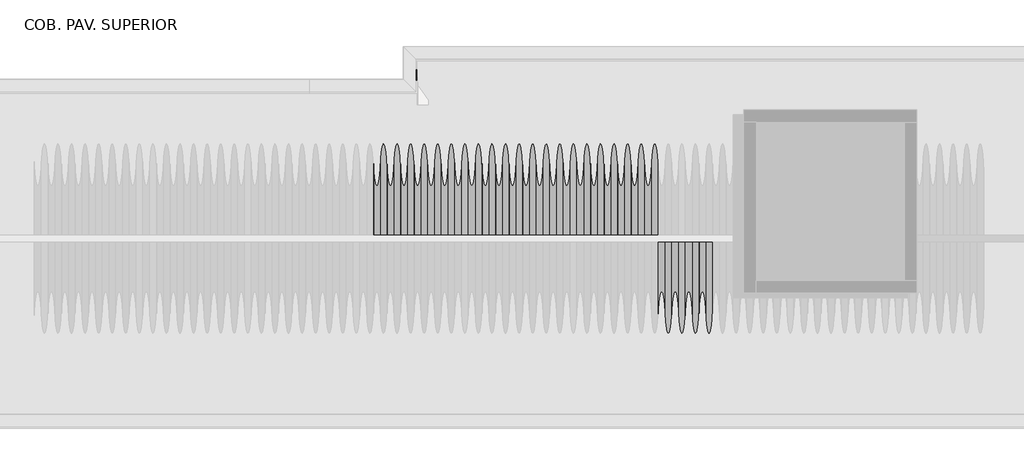
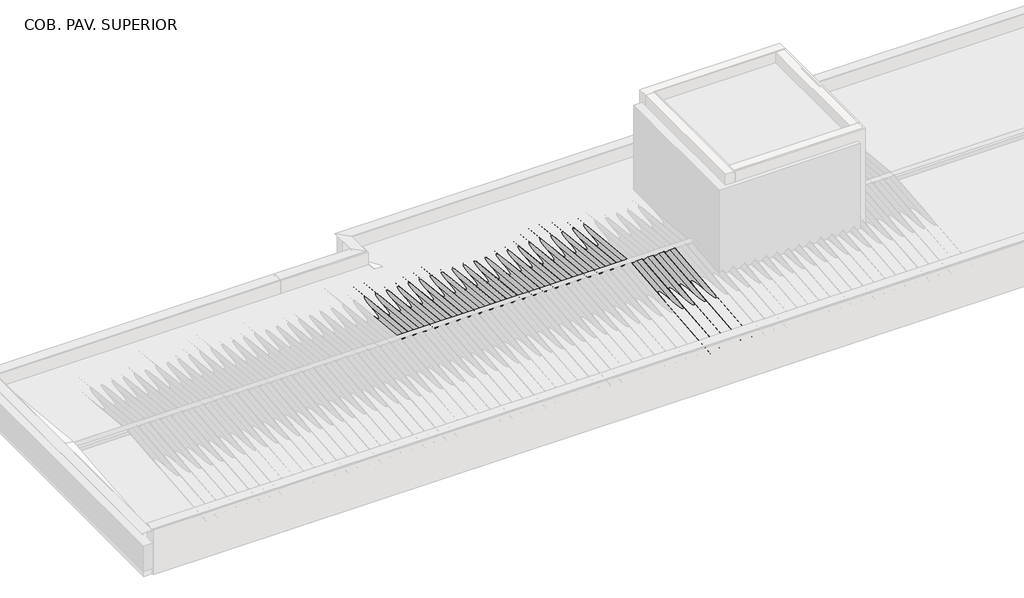
# One storey, part 5 of 8: 37 beams, 12 columns.
"""IFC4 building model written with IfcOpenShell, lengths in millimetres."""

import ifcopenshell
import ifcopenshell.guid

model = None  # the IFC model being written
_history = None  # IfcOwnerHistory: only IFC2X3 demands one
_inside = {}  # id of a spatial element -> (the spatial element, [elements in it])
_under = {}  # id of a project, library or spatial element -> (it, [spatial elements below it])
_declared = {}  # id of a project -> (the project, [libraries it declares])
_typed = {}  # id of a type object -> (the type object, [elements of that type])
_made_of = {}  # id of a material, layer set ... -> (it, [elements and type objects made of it])


def new_model(schema):
    """Start an empty IFC model of exactly this schema.

    Asked for "IFC4X3", IfcOpenShell would pick the latest addendum, in which some entities
    have other attributes; the version numbers below select the first issue.
    IFC2X3 requires an IfcOwnerHistory on every rooted entity: one is made here for all.
    """
    global model, _history
    if schema == "IFC4X3":
        model = ifcopenshell.file(schema_version=(4, 3, 0, 0))
    else:
        model = ifcopenshell.file(schema=schema)
    _inside.clear()
    _under.clear()
    _declared.clear()
    _typed.clear()
    _made_of.clear()
    _history = None
    if model.schema == "IFC2X3":
        org = make("IfcOrganization", Name="unknown")
        user = make(
            "IfcPersonAndOrganization",
            ThePerson=make("IfcPerson", FamilyName="unknown"),
            TheOrganization=org,
        )
        app = make(
            "IfcApplication",
            ApplicationDeveloper=org,
            Version="unknown",
            ApplicationFullName="unknown",
            ApplicationIdentifier="unknown",
        )
        _history = make(
            "IfcOwnerHistory",
            OwningUser=user,
            OwningApplication=app,
            ChangeAction="ADDED",
            CreationDate=0,
        )
    return model


def make(cls, **values):
    """One entity of the class cls with the attributes given. An attribute that is None is left unset."""
    return model.create_entity(
        cls, **{name: value for name, value in values.items() if value is not None}
    )


def rooted(cls, **values):
    """An entity with a GlobalId (a new one), such as an element, a storey or a relation."""
    return make(cls, GlobalId=ifcopenshell.guid.new(), OwnerHistory=_history, **values)


def si_unit(unit_type, name, prefix=None):
    """IfcSIUnit, for example si_unit("LENGTHUNIT", "METRE", prefix="MILLI")."""
    return make("IfcSIUnit", UnitType=unit_type, Prefix=prefix, Name=name)


def assignment(units):
    """IfcUnitAssignment: the units of a project."""
    return None if units is None else make("IfcUnitAssignment", Units=units)


def point(xyz):
    """IfcCartesianPoint."""
    return None if xyz is None else make("IfcCartesianPoint", Coordinates=xyz)


def direction(xyz):
    """IfcDirection."""
    return None if xyz is None else make("IfcDirection", DirectionRatios=xyz)


def frame(location, z_axis=None, x_axis=None):
    """IfcAxis2Placement3D, a coordinate frame: its origin and axes. An axis left out is left unset."""
    return make(
        "IfcAxis2Placement3D",
        Location=point(location),
        Axis=direction(z_axis),
        RefDirection=direction(x_axis),
    )


def frame_2d(location, x_axis=None):
    """IfcAxis2Placement2D, a coordinate frame in the plane: its origin and x axis."""
    return make(
        "IfcAxis2Placement2D", Location=point(location), RefDirection=direction(x_axis)
    )


def origin():
    """The frame at (0, 0, 0) with its axes left unset."""
    return frame((0.0, 0.0, 0.0))


def place(relative_to, where):
    """IfcLocalPlacement: puts the frame where relative to a parent placement (None: the world)."""
    return make(
        "IfcLocalPlacement", PlacementRelTo=relative_to, RelativePlacement=where
    )


def context(
    kind, dimensions, precision=None, world=None, true_north=None, identifier=None
):
    """IfcGeometricRepresentationContext, for example the 3D "Model" context."""
    return make(
        "IfcGeometricRepresentationContext",
        ContextIdentifier=identifier,
        ContextType=kind,
        CoordinateSpaceDimension=dimensions,
        Precision=precision,
        WorldCoordinateSystem=world,
        TrueNorth=true_north,
    )


def project(units=None, contexts=None):
    """IfcProject with its units and contexts."""
    return rooted(
        "IfcProject",
        Name="project",
        RepresentationContexts=contexts,
        UnitsInContext=assignment(units),
    )


def spatial(cls, under=None, at=None, **own):
    """A site, building, storey or space (cls), placed at a placement, below another one or the project."""
    s = rooted(cls, ObjectPlacement=at, **own)
    if under is not None:
        _under.setdefault(under.id(), (under, []))[1].append(s)
    return s


def polyline(points):
    """IfcPolyline through the points."""
    return make("IfcPolyline", Points=[point(p) for p in points])


def circle_curve(where, radius):
    """IfcCircle in the frame where."""
    return make("IfcCircle", Position=where, Radius=radius)


def trimmed(basis, trim1, trim2, sense, master):
    """IfcTrimmedCurve: the piece of a basis curve between two trims."""
    return make(
        "IfcTrimmedCurve",
        BasisCurve=basis,
        Trim1=trim1,
        Trim2=trim2,
        SenseAgreement=sense,
        MasterRepresentation=master,
    )


def segment(curve, same_sense, transition):
    """IfcCompositeCurveSegment."""
    return make(
        "IfcCompositeCurveSegment",
        Transition=transition,
        SameSense=same_sense,
        ParentCurve=curve,
    )


def composite_curve(segments, self_intersect=None):
    """IfcCompositeCurve: segments joined end to end."""
    return make("IfcCompositeCurve", Segments=segments, SelfIntersect=self_intersect)


def outline(outer, holes=None, kind="AREA"):
    """IfcArbitraryClosedProfileDef: a profile drawn as a closed curve; with holes, ...WithVoids."""
    if holes is None:
        return make("IfcArbitraryClosedProfileDef", ProfileType=kind, OuterCurve=outer)
    return make(
        "IfcArbitraryProfileDefWithVoids",
        ProfileType=kind,
        OuterCurve=outer,
        InnerCurves=holes,
    )


def extrude(swept, where, along, depth):
    """IfcExtrudedAreaSolid: the profile swept, set in the frame where, extruded along a direction by depth."""
    return make(
        "IfcExtrudedAreaSolid",
        SweptArea=swept,
        Position=where,
        ExtrudedDirection=direction(along),
        Depth=depth,
    )


def shape(context_of_items, identifier, shape_type, items):
    """IfcShapeRepresentation: the items that make up one representation, for example the "Body"."""
    return make(
        "IfcShapeRepresentation",
        ContextOfItems=context_of_items,
        RepresentationIdentifier=identifier,
        RepresentationType=shape_type,
        Items=items,
    )


def source(mapping_origin, context_of_items, identifier, shape_type, items):
    """IfcRepresentationMap: a shape defined once, which mapped items show again and again."""
    return make(
        "IfcRepresentationMap",
        MappingOrigin=mapping_origin,
        MappedRepresentation=shape(context_of_items, identifier, shape_type, items),
    )


def transform(
    local_origin,
    x_axis=None,
    y_axis=None,
    z_axis=None,
    scale=None,
    scale2=None,
    scale3=None,
    uniform=True,
):
    """IfcCartesianTransformationOperator3D, or its non-uniform kind. x_axis, y_axis, z_axis: its Axis1, 2, 3."""
    if uniform:
        return make(
            "IfcCartesianTransformationOperator3D",
            Axis1=direction(x_axis),
            Axis2=direction(y_axis),
            LocalOrigin=point(local_origin),
            Scale=scale,
            Axis3=direction(z_axis),
        )
    return make(
        "IfcCartesianTransformationOperator3DnonUniform",
        Axis1=direction(x_axis),
        Axis2=direction(y_axis),
        LocalOrigin=point(local_origin),
        Scale=scale,
        Axis3=direction(z_axis),
        Scale2=scale2,
        Scale3=scale3,
    )


def mapped(mapping_source, mapping_target):
    """IfcMappedItem: shows the shape of a source again, moved by a transform."""
    return make(
        "IfcMappedItem", MappingSource=mapping_source, MappingTarget=mapping_target
    )


def made_of(thing, what):
    """Note that an element or type object is made of a material, layer set ...; save() writes the relation."""
    if what is not None:
        _made_of.setdefault(what.id(), (what, []))[1].append(thing)
    return thing


def element(
    cls,
    number,
    at=None,
    inside=None,
    cuts=None,
    type_object=None,
    material=None,
    context=None,
    identifier="Body",
    shape_type=None,
    held_by="IfcProductDefinitionShape",
    body=None,
    shapes=None,
    **own,
):
    """One element of the class cls, such as IfcWall. Its Tag is "e" and its number.

    at: its placement. inside: the storey or other place that contains it. cuts: it is an
    opening in that element (IfcRelVoidsElement). A single representation is given by context,
    identifier, shape_type and body (its items); several are given by shapes. held_by: the class
    of the entity that holds the representations. save() writes the other relations.
    """
    e = rooted(cls, Tag="e%d" % number, ObjectPlacement=at, **own)
    if body is not None:
        shapes = [shape(context, identifier, shape_type, body)]
    if shapes is not None:
        e.Representation = make(held_by, Representations=shapes)
    if inside is not None:
        _inside.setdefault(inside.id(), (inside, []))[1].append(e)
    if cuts is not None:
        rooted(
            "IfcRelVoidsElement", RelatingBuildingElement=cuts, RelatedOpeningElement=e
        )
    if type_object is not None:
        _typed.setdefault(type_object.id(), (type_object, []))[1].append(e)
    return made_of(e, material)


def aggregate(whole, parts):
    """IfcRelAggregates: a whole, such as a stair, and the parts it consists of."""
    return rooted("IfcRelAggregates", RelatingObject=whole, RelatedObjects=parts)


def save(model, path):
    """Write the relations noted so far, then the file.

    IfcRelAggregates (storeys below a building ...), IfcRelContainedInSpatialStructure (elements
    in a storey), IfcRelDefinesByType, IfcRelAssociatesMaterial and IfcRelDeclares: one each for
    every whole, place, type object, material and project.
    """
    for whole, parts in _under.values():
        aggregate(whole, parts)
    for where, things in _inside.values():
        rooted(
            "IfcRelContainedInSpatialStructure",
            RelatedElements=things,
            RelatingStructure=where,
        )
    for kind, things in _typed.values():
        rooted("IfcRelDefinesByType", RelatedObjects=things, RelatingType=kind)
    for what, things in _made_of.values():
        rooted("IfcRelAssociatesMaterial", RelatedObjects=things, RelatingMaterial=what)
    for by, libraries in _declared.values():
        rooted("IfcRelDeclares", RelatingContext=by, RelatedDefinitions=libraries)
    model.write(path)


def beam_fe4ddbad(model_context):
    return source(origin(), model_context, "Body", "SweptSolid", [
        extrude(outline(polyline([(998.8971968, 30.0), (998.8971968, -30.0), (-998.8971974, -30.0), (-998.8971974, 30.0), (998.8971968, 30.0)])), frame((0.0, 0.0, -60.0), z_axis=(0.0, 0.0, 1.0), x_axis=(1.0, 0.0, 0.0)), (0.0, 0.0, 1.0), 120.0),
    ])


def beam_739eac5c(model_context):
    return source(origin(), model_context, "Body", "SweptSolid", [
        extrude(outline(polyline([(854.9999994, 30.0), (854.9999994, -30.0), (-855.0, -30.0), (-855.0, 30.0), (854.9999994, 30.0)])), frame((0.0, 0.0, -60.0), z_axis=(0.0, 0.0, 1.0), x_axis=(1.0, 0.0, 0.0)), (0.0, 0.0, 1.0), 120.0),
    ])


def beam_e1aa0c85(model_context):
    return source(origin(), model_context, "Body", "SweptSolid", [
        extrude(outline(polyline([(144.2686794, 30.0), (144.2686794, -30.0), (-144.2686794, -30.0), (-144.2686794, 30.0), (144.2686794, 30.0)])), frame((0.0, 0.0, -60.0), z_axis=(0.0, 0.0, 1.0), x_axis=(1.0, 0.0, 0.0)), (0.0, 0.0, 1.0), 120.0),
    ])


def column_6c15bf79(model_context):
    return source(origin(), model_context, "Body", "SweptSolid", [
        extrude(outline(polyline([(30.0, 80.0), (30.0, -80.0), (-30.0, -80.0), (-30.0, 80.0), (30.0, 80.0)])), frame((0.0, 0.0, 6710.0), z_axis=(0.0, 0.0, 1.0), x_axis=(1.0, 0.0, 0.0)), (0.0, 0.0, 1.0), 467.5),
    ])


def column_1adb463a(model_context):
    return source(origin(), model_context, "Body", "SweptSolid", [
        extrude(outline(polyline([(30.0, 80.0), (30.0, -80.0), (-30.0, -80.0), (-30.0, 80.0), (30.0, 80.0)])), frame((0.0, 0.0, 6710.0), z_axis=(0.0, 0.0, 1.0), x_axis=(1.0, 0.0, 0.0)), (0.0, 0.0, 1.0), 284.6),
    ])


def column_910cb117(model_context):
    return source(origin(), model_context, "Body", "SweptSolid", [
        extrude(outline(polyline([(30.0, 80.0), (30.0, -80.0), (-30.0, -80.0), (-30.0, 80.0), (30.0, 80.0)])), frame((0.0, 0.0, 6710.0), z_axis=(0.0, 0.0, 1.0), x_axis=(1.0, 0.0, 0.0)), (0.0, 0.0, 1.0), 371.3),
    ])


def column_42eef9f8(model_context):
    return source(origin(), model_context, "Body", "SweptSolid", [
        extrude(outline(polyline([(30.0, 80.0), (30.0, -80.0), (-30.0, -80.0), (-30.0, 80.0), (30.0, 80.0)])), frame((0.0, 0.0, 6710.0), z_axis=(0.0, 0.0, 1.0), x_axis=(1.0, 0.0, 0.0)), (0.0, 0.0, 1.0), 227.1),
    ])


model = new_model("IFC4")

# Units and contexts
model_context = context("Model", 3, world=origin())
ifc_project = project(units=[si_unit("LENGTHUNIT", "METRE", prefix="MILLI")], contexts=[model_context])

# Site, building, storey
site = spatial("IfcSite", under=ifc_project)
building = spatial("IfcBuilding", under=site)
storey = spatial("IfcBuildingStorey", under=building, Name="COB. PAV. SUPERIOR", Elevation=6650.0)

# Beams
placement = place(None, origin())
beam_shape = beam_fe4ddbad(model_context)
element("IfcBeam", 1, ObjectType="Madeira de lei : Berço 6x12cm", at=placement, inside=storey, context=model_context, shape_type="MappedRepresentation", body=[
    mapped(beam_shape, transform((-3747.0065303, -7777.6209418, 6680.0), x_axis=(1.0, 0.0, 0.0), y_axis=(0.0, 0.0, -1.0), z_axis=(0.0, 1.0, 0.0))),
])
element("IfcBeam", 2, ObjectType="Madeira de lei : Berço 6x12cm", at=placement, inside=storey, context=model_context, shape_type="MappedRepresentation", body=[
    mapped(beam_shape, transform((-1749.2121355, -7777.6209418, 6680.0), x_axis=(1.0, 0.0, 0.0), y_axis=(0.0, 0.0, -1.0), z_axis=(0.0, 1.0, 0.0))),
])
element("IfcBeam", 3, ObjectType="Madeira de lei : Berço 6x12cm", at=placement, inside=storey, context=model_context, shape_type="MappedRepresentation", body=[
    mapped(beam_shape, transform((-5744.8009251, -6365.3711004, 6680.0), x_axis=(1.0, 0.0, 0.0), y_axis=(0.0, 0.0, -1.0), z_axis=(0.0, 1.0, 0.0))),
])
element("IfcBeam", 4, ObjectType="Madeira de lei : Berço 6x12cm", at=placement, inside=storey, context=model_context, shape_type="MappedRepresentation", body=[
    mapped(beam_shape, transform((-3747.0065303, -6365.3711004, 6680.0), x_axis=(1.0, 0.0, 0.0), y_axis=(0.0, 0.0, -1.0), z_axis=(0.0, 1.0, 0.0))),
])
element("IfcBeam", 5, ObjectType="Madeira de lei : Berço 6x12cm", at=placement, inside=storey, context=model_context, shape_type="MappedRepresentation", body=[
    mapped(beam_shape, transform((-1749.2121355, -6365.3711004, 6680.0), x_axis=(1.0, 0.0, 0.0), y_axis=(0.0, 0.0, -1.0), z_axis=(0.0, 1.0, 0.0))),
])
element("IfcBeam", 6, ObjectType="Madeira de lei : Berço 6x12cm", at=placement, inside=storey, context=model_context, shape_type="MappedRepresentation", body=[
    mapped(beam_shape, transform((-7742.5953199, -5498.3211004, 6680.0), x_axis=(1.0, 0.0, 0.0), y_axis=(0.0, 0.0, -1.0), z_axis=(0.0, 1.0, 0.0))),
])
element("IfcBeam", 7, ObjectType="Madeira de lei : Berço 6x12cm", at=placement, inside=storey, context=model_context, shape_type="MappedRepresentation", body=[
    mapped(beam_shape, transform((-5744.8009251, -5498.3211004, 6680.0), x_axis=(1.0, 0.0, 0.0), y_axis=(0.0, 0.0, -1.0), z_axis=(0.0, 1.0, 0.0))),
])
element("IfcBeam", 8, ObjectType="Madeira de lei : Berço 6x12cm", at=placement, inside=storey, context=model_context, shape_type="MappedRepresentation", body=[
    mapped(beam_shape, transform((248.5822594, -10631.818869, 6680.0), x_axis=(1.0, 0.0, 0.0), y_axis=(0.0, 0.0, -1.0), z_axis=(0.0, 1.0, 0.0))),
])
element("IfcBeam", 9, ObjectType="Madeira de lei : Berço 6x12cm", at=placement, inside=storey, context=model_context, shape_type="MappedRepresentation", body=[
    mapped(beam_shape, transform((2246.3766542, -10631.818869, 6680.0), x_axis=(1.0, 0.0, 0.0), y_axis=(0.0, 0.0, -1.0), z_axis=(0.0, 1.0, 0.0))),
])
element("IfcBeam", 10, ObjectType="Madeira de lei : Berço 6x12cm", at=placement, inside=storey, context=model_context, shape_type="MappedRepresentation", body=[
    mapped(beam_shape, transform((-1749.2121327, -4923.3211004, 6680.0), x_axis=(1.0, 0.0, 0.0), y_axis=(0.0, 0.0, -1.0), z_axis=(0.0, 1.0, 0.0))),
])
beam_2_shape = beam_739eac5c(model_context)
element("IfcBeam", 11, ObjectType="Madeira de lei : Berço 6x12cm", at=placement, inside=storey, context=model_context, shape_type="MappedRepresentation", body=[
    mapped(beam_2_shape, transform((-3603.1093298, -4923.3211004, 6680.0), x_axis=(1.0, 0.0, 0.0), y_axis=(0.0, 0.0, -1.0), z_axis=(0.0, 1.0, 0.0))),
])
beam_3_shape = beam_e1aa0c85(model_context)
element("IfcBeam", 12, ObjectType="Madeira de lei : Berço 6x12cm", at=placement, inside=storey, context=model_context, shape_type="MappedRepresentation", body=[
    mapped(beam_3_shape, transform((-4601.6350482, -5498.3211004, 6680.0), x_axis=(1.0, 0.0, 0.0), y_axis=(0.0, 0.0, -1.0), z_axis=(0.0, 1.0, 0.0))),
])
element("IfcBeam", 13, ObjectType="Telha Ondulada : Fibrocimento", at=placement, inside=storey, context=model_context, shape_type="SweptSolid", body=[
    extrude(outline(composite_curve([segment(trimmed(circle_curve(frame_2d((0.0, 66.7939461)), 66.7939461), [point((29.3501489, 6.7939461))], [point((29.3501489, 126.7939461))], True, "CARTESIAN"), True, "CONTINUOUS"), segment(polyline([(29.3501489, 126.7939461), (31.5472154, 131.2853711)]), True, "CONTINUOUS"), segment(trimmed(circle_curve(frame_2d((0.0, 66.7939461)), 71.7939461), [point((31.5472154, 131.2853711))], [point((31.5472154, 2.3025211))], False, "CARTESIAN"), True, "CONTINUOUS"), segment(trimmed(circle_curve(frame_2d((58.7002978, -53.2060539)), 61.7939461), [point((31.5472154, 2.3025211))], [point((31.5472154, -108.7146289))], True, "CARTESIAN"), True, "CONTINUOUS"), segment(polyline([(31.5472154, -108.7146289), (29.3501489, -113.2060539)]), True, "CONTINUOUS"), segment(trimmed(circle_curve(frame_2d((58.7002978, -53.2060539)), 66.7939461), [point((29.3501489, -113.2060539))], [point((29.3501489, 6.7939461))], False, "CARTESIAN"), True, "CONTINUOUS")], self_intersect=False)), frame((16.7156257, -10831.9594023, 7106.8215886), z_axis=(0.0, 0.9950371902099894, 0.09950371902099749), x_axis=(0.0, 0.09950371902099749, -0.9950371902099894)), (0.0, 0.0, 1.0), 3060.4439799),
])
element("IfcBeam", 14, ObjectType="Telha Ondulada : Fibrocimento", at=placement, inside=storey, context=model_context, shape_type="SweptSolid", body=[
    extrude(outline(composite_curve([segment(trimmed(circle_curve(frame_2d((0.0, 66.7939461)), 66.7939461), [point((29.3501489, 6.7939461))], [point((29.3501489, 126.7939461))], True, "CARTESIAN"), True, "CONTINUOUS"), segment(polyline([(29.3501489, 126.7939461), (31.5472154, 131.2853711)]), True, "CONTINUOUS"), segment(trimmed(circle_curve(frame_2d((0.0, 66.7939461)), 71.7939461), [point((31.5472154, 131.2853711))], [point((31.5472154, 2.3025211))], False, "CARTESIAN"), True, "CONTINUOUS"), segment(trimmed(circle_curve(frame_2d((58.7002978, -53.2060539)), 61.7939461), [point((31.5472154, 2.3025211))], [point((31.5472154, -108.7146289))], True, "CARTESIAN"), True, "CONTINUOUS"), segment(polyline([(31.5472154, -108.7146289), (29.3501489, -113.2060539)]), True, "CONTINUOUS"), segment(trimmed(circle_curve(frame_2d((58.7002978, -53.2060539)), 66.7939461), [point((29.3501489, -113.2060539))], [point((29.3501489, 6.7939461))], False, "CARTESIAN"), True, "CONTINUOUS")], self_intersect=False)), frame((261.2156257, -10831.9594023, 7106.8215886), z_axis=(0.0, 0.9950371902099894, 0.09950371902099749), x_axis=(0.0, 0.09950371902099749, -0.9950371902099894)), (0.0, 0.0, 1.0), 3060.4439799),
])
element("IfcBeam", 15, ObjectType="Telha Ondulada : Fibrocimento", at=placement, inside=storey, context=model_context, shape_type="SweptSolid", body=[
    extrude(outline(composite_curve([segment(trimmed(circle_curve(frame_2d((0.0, 66.7939461)), 66.7939461), [point((29.3501489, 6.7939461))], [point((29.3501489, 126.7939461))], True, "CARTESIAN"), True, "CONTINUOUS"), segment(polyline([(29.3501489, 126.7939461), (31.5472154, 131.2853711)]), True, "CONTINUOUS"), segment(trimmed(circle_curve(frame_2d((0.0, 66.7939461)), 71.7939461), [point((31.5472154, 131.2853711))], [point((31.5472154, 2.3025211))], False, "CARTESIAN"), True, "CONTINUOUS"), segment(trimmed(circle_curve(frame_2d((58.7002978, -53.2060539)), 61.7939461), [point((31.5472154, 2.3025211))], [point((31.5472154, -108.7146289))], True, "CARTESIAN"), True, "CONTINUOUS"), segment(polyline([(31.5472154, -108.7146289), (29.3501489, -113.2060539)]), True, "CONTINUOUS"), segment(trimmed(circle_curve(frame_2d((58.7002978, -53.2060539)), 66.7939461), [point((29.3501489, -113.2060539))], [point((29.3501489, 6.7939461))], False, "CARTESIAN"), True, "CONTINUOUS")], self_intersect=False)), frame((505.7156257, -10831.9594023, 7106.8215886), z_axis=(0.0, 0.9950371902099894, 0.09950371902099749), x_axis=(0.0, 0.09950371902099749, -0.9950371902099894)), (0.0, 0.0, 1.0), 3060.4439799),
])
element("IfcBeam", 16, ObjectType="Telha Ondulada : Fibrocimento", at=placement, inside=storey, context=model_context, shape_type="SweptSolid", body=[
    extrude(outline(composite_curve([segment(trimmed(circle_curve(frame_2d((0.0, 66.7939461)), 66.7939461), [point((29.3501489, 6.7939461))], [point((29.3501489, 126.7939461))], True, "CARTESIAN"), True, "CONTINUOUS"), segment(polyline([(29.3501489, 126.7939461), (31.5472154, 131.2853711)]), True, "CONTINUOUS"), segment(trimmed(circle_curve(frame_2d((0.0, 66.7939461)), 71.7939461), [point((31.5472154, 131.2853711))], [point((31.5472154, 2.3025211))], False, "CARTESIAN"), True, "CONTINUOUS"), segment(trimmed(circle_curve(frame_2d((58.7002978, -53.2060539)), 61.7939461), [point((31.5472154, 2.3025211))], [point((31.5472154, -108.7146289))], True, "CARTESIAN"), True, "CONTINUOUS"), segment(polyline([(31.5472154, -108.7146289), (29.3501489, -113.2060539)]), True, "CONTINUOUS"), segment(trimmed(circle_curve(frame_2d((58.7002978, -53.2060539)), 66.7939461), [point((29.3501489, -113.2060539))], [point((29.3501489, 6.7939461))], False, "CARTESIAN"), True, "CONTINUOUS")], self_intersect=False)), frame((750.2156257, -10831.9594023, 7106.8215886), z_axis=(0.0, 0.9950371902099894, 0.09950371902099749), x_axis=(0.0, 0.09950371902099749, -0.9950371902099894)), (0.0, 0.0, 1.0), 3060.4439799),
])
element("IfcBeam", 17, ObjectType="Telha Ondulada : Fibrocimento", at=placement, inside=storey, context=model_context, shape_type="SweptSolid", body=[
    extrude(outline(composite_curve([segment(trimmed(circle_curve(frame_2d((-58.7002978, -53.2060539)), 66.7939461), [point((-29.3501489, 6.7939461))], [point((-29.3501489, -113.2060539))], False, "CARTESIAN"), True, "CONTINUOUS"), segment(polyline([(-29.3501489, -113.2060539), (-31.5472154, -108.7146289)]), True, "CONTINUOUS"), segment(trimmed(circle_curve(frame_2d((-58.7002978, -53.2060539)), 61.7939461), [point((-31.5472154, -108.7146289))], [point((-31.5472154, 2.3025211))], True, "CARTESIAN"), True, "CONTINUOUS"), segment(trimmed(circle_curve(frame_2d((0.0, 66.7939461)), 71.7939461), [point((-31.5472154, 2.3025211))], [point((-31.5472154, 131.2853711))], False, "CARTESIAN"), True, "CONTINUOUS"), segment(polyline([(-31.5472154, 131.2853711), (-29.3501489, 126.7939461)]), True, "CONTINUOUS"), segment(trimmed(circle_curve(frame_2d((0.0, 66.7939461)), 66.7939461), [point((-29.3501489, 126.7939461))], [point((-29.3501489, 6.7939461))], True, "CARTESIAN"), True, "CONTINUOUS")], self_intersect=False)), frame((-5117.7843743, -5298.1805671, 7164.3215886), z_axis=(0.0, -0.9950371902099894, 0.09950371902099785), x_axis=(0.0, 0.09950371902099785, 0.9950371902099894)), (0.0, 0.0, 1.0), 2482.5761317),
])
element("IfcBeam", 18, ObjectType="Telha Ondulada : Fibrocimento", at=placement, inside=storey, context=model_context, shape_type="SweptSolid", body=[
    extrude(outline(composite_curve([segment(trimmed(circle_curve(frame_2d((-58.7002978, -53.2060539)), 66.7939461), [point((-29.3501489, 6.7939461))], [point((-29.3501489, -113.2060539))], False, "CARTESIAN"), True, "CONTINUOUS"), segment(polyline([(-29.3501489, -113.2060539), (-31.5472154, -108.7146289)]), True, "CONTINUOUS"), segment(trimmed(circle_curve(frame_2d((-58.7002978, -53.2060539)), 61.7939461), [point((-31.5472154, -108.7146289))], [point((-31.5472154, 2.3025211))], True, "CARTESIAN"), True, "CONTINUOUS"), segment(trimmed(circle_curve(frame_2d((0.0, 66.7939461)), 71.7939461), [point((-31.5472154, 2.3025211))], [point((-31.5472154, 131.2853711))], False, "CARTESIAN"), True, "CONTINUOUS"), segment(polyline([(-31.5472154, 131.2853711), (-29.3501489, 126.7939461)]), True, "CONTINUOUS"), segment(trimmed(circle_curve(frame_2d((0.0, 66.7939461)), 66.7939461), [point((-29.3501489, 126.7939461))], [point((-29.3501489, 6.7939461))], True, "CARTESIAN"), True, "CONTINUOUS")], self_intersect=False)), frame((-4873.2843743, -5298.1805671, 7164.3215886), z_axis=(0.0, -0.9950371902099894, 0.09950371902099785), x_axis=(0.0, 0.09950371902099785, 0.9950371902099894)), (0.0, 0.0, 1.0), 2482.5761317),
])
element("IfcBeam", 19, ObjectType="Telha Ondulada : Fibrocimento", at=placement, inside=storey, context=model_context, shape_type="SweptSolid", body=[
    extrude(outline(composite_curve([segment(trimmed(circle_curve(frame_2d((-58.7002978, -53.2060539)), 66.7939461), [point((-29.3501489, 6.7939461))], [point((-29.3501489, -113.2060539))], False, "CARTESIAN"), True, "CONTINUOUS"), segment(polyline([(-29.3501489, -113.2060539), (-31.5472154, -108.7146289)]), True, "CONTINUOUS"), segment(trimmed(circle_curve(frame_2d((-58.7002978, -53.2060539)), 61.7939461), [point((-31.5472154, -108.7146289))], [point((-31.5472154, 2.3025211))], True, "CARTESIAN"), True, "CONTINUOUS"), segment(trimmed(circle_curve(frame_2d((0.0, 66.7939461)), 71.7939461), [point((-31.5472154, 2.3025211))], [point((-31.5472154, 131.2853711))], False, "CARTESIAN"), True, "CONTINUOUS"), segment(polyline([(-31.5472154, 131.2853711), (-29.3501489, 126.7939461)]), True, "CONTINUOUS"), segment(trimmed(circle_curve(frame_2d((0.0, 66.7939461)), 66.7939461), [point((-29.3501489, 126.7939461))], [point((-29.3501489, 6.7939461))], True, "CARTESIAN"), True, "CONTINUOUS")], self_intersect=False)), frame((-4628.7843743, -5298.1805671, 7164.3215886), z_axis=(0.0, -0.9950371902099894, 0.09950371902099785), x_axis=(0.0, 0.09950371902099785, 0.9950371902099894)), (0.0, 0.0, 1.0), 2482.5761317),
])
element("IfcBeam", 20, ObjectType="Telha Ondulada : Fibrocimento", at=placement, inside=storey, context=model_context, shape_type="SweptSolid", body=[
    extrude(outline(composite_curve([segment(trimmed(circle_curve(frame_2d((-58.7002978, -53.2060539)), 66.7939461), [point((-29.3501489, 6.7939461))], [point((-29.3501489, -113.2060539))], False, "CARTESIAN"), True, "CONTINUOUS"), segment(polyline([(-29.3501489, -113.2060539), (-31.5472154, -108.7146289)]), True, "CONTINUOUS"), segment(trimmed(circle_curve(frame_2d((-58.7002978, -53.2060539)), 61.7939461), [point((-31.5472154, -108.7146289))], [point((-31.5472154, 2.3025211))], True, "CARTESIAN"), True, "CONTINUOUS"), segment(trimmed(circle_curve(frame_2d((0.0, 66.7939461)), 71.7939461), [point((-31.5472154, 2.3025211))], [point((-31.5472154, 131.2853711))], False, "CARTESIAN"), True, "CONTINUOUS"), segment(polyline([(-31.5472154, 131.2853711), (-29.3501489, 126.7939461)]), True, "CONTINUOUS"), segment(trimmed(circle_curve(frame_2d((0.0, 66.7939461)), 66.7939461), [point((-29.3501489, 126.7939461))], [point((-29.3501489, 6.7939461))], True, "CARTESIAN"), True, "CONTINUOUS")], self_intersect=False)), frame((-4384.2843743, -4723.1805671, 7106.8215886), z_axis=(0.0, -0.9950371902099893, 0.09950371902099797), x_axis=(0.0, 0.09950371902099797, 0.9950371902099893)), (0.0, 0.0, 1.0), 3060.4439799),
])
element("IfcBeam", 21, ObjectType="Telha Ondulada : Fibrocimento", at=placement, inside=storey, context=model_context, shape_type="SweptSolid", body=[
    extrude(outline(composite_curve([segment(trimmed(circle_curve(frame_2d((-58.7002978, -53.2060539)), 66.7939461), [point((-29.3501489, 6.7939461))], [point((-29.3501489, -113.2060539))], False, "CARTESIAN"), True, "CONTINUOUS"), segment(polyline([(-29.3501489, -113.2060539), (-31.5472154, -108.7146289)]), True, "CONTINUOUS"), segment(trimmed(circle_curve(frame_2d((-58.7002978, -53.2060539)), 61.7939461), [point((-31.5472154, -108.7146289))], [point((-31.5472154, 2.3025211))], True, "CARTESIAN"), True, "CONTINUOUS"), segment(trimmed(circle_curve(frame_2d((0.0, 66.7939461)), 71.7939461), [point((-31.5472154, 2.3025211))], [point((-31.5472154, 131.2853711))], False, "CARTESIAN"), True, "CONTINUOUS"), segment(polyline([(-31.5472154, 131.2853711), (-29.3501489, 126.7939461)]), True, "CONTINUOUS"), segment(trimmed(circle_curve(frame_2d((0.0, 66.7939461)), 66.7939461), [point((-29.3501489, 126.7939461))], [point((-29.3501489, 6.7939461))], True, "CARTESIAN"), True, "CONTINUOUS")], self_intersect=False)), frame((-4139.7843743, -4723.1805671, 7106.8215886), z_axis=(0.0, -0.9950371902099893, 0.09950371902099797), x_axis=(0.0, 0.09950371902099797, 0.9950371902099893)), (0.0, 0.0, 1.0), 3060.4439799),
])
element("IfcBeam", 22, ObjectType="Telha Ondulada : Fibrocimento", at=placement, inside=storey, context=model_context, shape_type="SweptSolid", body=[
    extrude(outline(composite_curve([segment(trimmed(circle_curve(frame_2d((-58.7002978, -53.2060539)), 66.7939461), [point((-29.3501489, 6.7939461))], [point((-29.3501489, -113.2060539))], False, "CARTESIAN"), True, "CONTINUOUS"), segment(polyline([(-29.3501489, -113.2060539), (-31.5472154, -108.7146289)]), True, "CONTINUOUS"), segment(trimmed(circle_curve(frame_2d((-58.7002978, -53.2060539)), 61.7939461), [point((-31.5472154, -108.7146289))], [point((-31.5472154, 2.3025211))], True, "CARTESIAN"), True, "CONTINUOUS"), segment(trimmed(circle_curve(frame_2d((0.0, 66.7939461)), 71.7939461), [point((-31.5472154, 2.3025211))], [point((-31.5472154, 131.2853711))], False, "CARTESIAN"), True, "CONTINUOUS"), segment(polyline([(-31.5472154, 131.2853711), (-29.3501489, 126.7939461)]), True, "CONTINUOUS"), segment(trimmed(circle_curve(frame_2d((0.0, 66.7939461)), 66.7939461), [point((-29.3501489, 126.7939461))], [point((-29.3501489, 6.7939461))], True, "CARTESIAN"), True, "CONTINUOUS")], self_intersect=False)), frame((-3895.2843743, -4723.1805671, 7106.8215886), z_axis=(0.0, -0.9950371902099893, 0.09950371902099797), x_axis=(0.0, 0.09950371902099797, 0.9950371902099893)), (0.0, 0.0, 1.0), 3060.4439799),
])
element("IfcBeam", 23, ObjectType="Telha Ondulada : Fibrocimento", at=placement, inside=storey, context=model_context, shape_type="SweptSolid", body=[
    extrude(outline(composite_curve([segment(trimmed(circle_curve(frame_2d((-58.7002978, -53.2060539)), 66.7939461), [point((-29.3501489, 6.7939461))], [point((-29.3501489, -113.2060539))], False, "CARTESIAN"), True, "CONTINUOUS"), segment(polyline([(-29.3501489, -113.2060539), (-31.5472154, -108.7146289)]), True, "CONTINUOUS"), segment(trimmed(circle_curve(frame_2d((-58.7002978, -53.2060539)), 61.7939461), [point((-31.5472154, -108.7146289))], [point((-31.5472154, 2.3025211))], True, "CARTESIAN"), True, "CONTINUOUS"), segment(trimmed(circle_curve(frame_2d((0.0, 66.7939461)), 71.7939461), [point((-31.5472154, 2.3025211))], [point((-31.5472154, 131.2853711))], False, "CARTESIAN"), True, "CONTINUOUS"), segment(polyline([(-31.5472154, 131.2853711), (-29.3501489, 126.7939461)]), True, "CONTINUOUS"), segment(trimmed(circle_curve(frame_2d((0.0, 66.7939461)), 66.7939461), [point((-29.3501489, 126.7939461))], [point((-29.3501489, 6.7939461))], True, "CARTESIAN"), True, "CONTINUOUS")], self_intersect=False)), frame((-3650.7843743, -4723.1805671, 7106.8215886), z_axis=(0.0, -0.9950371902099893, 0.09950371902099797), x_axis=(0.0, 0.09950371902099797, 0.9950371902099893)), (0.0, 0.0, 1.0), 3060.4439799),
])
element("IfcBeam", 24, ObjectType="Telha Ondulada : Fibrocimento", at=placement, inside=storey, context=model_context, shape_type="SweptSolid", body=[
    extrude(outline(composite_curve([segment(trimmed(circle_curve(frame_2d((-58.7002978, -53.2060539)), 66.7939461), [point((-29.3501489, 6.7939461))], [point((-29.3501489, -113.2060539))], False, "CARTESIAN"), True, "CONTINUOUS"), segment(polyline([(-29.3501489, -113.2060539), (-31.5472154, -108.7146289)]), True, "CONTINUOUS"), segment(trimmed(circle_curve(frame_2d((-58.7002978, -53.2060539)), 61.7939461), [point((-31.5472154, -108.7146289))], [point((-31.5472154, 2.3025211))], True, "CARTESIAN"), True, "CONTINUOUS"), segment(trimmed(circle_curve(frame_2d((0.0, 66.7939461)), 71.7939461), [point((-31.5472154, 2.3025211))], [point((-31.5472154, 131.2853711))], False, "CARTESIAN"), True, "CONTINUOUS"), segment(polyline([(-31.5472154, 131.2853711), (-29.3501489, 126.7939461)]), True, "CONTINUOUS"), segment(trimmed(circle_curve(frame_2d((0.0, 66.7939461)), 66.7939461), [point((-29.3501489, 126.7939461))], [point((-29.3501489, 6.7939461))], True, "CARTESIAN"), True, "CONTINUOUS")], self_intersect=False)), frame((-3406.2843743, -4723.1805671, 7106.8215886), z_axis=(0.0, -0.9950371902099893, 0.09950371902099797), x_axis=(0.0, 0.09950371902099797, 0.9950371902099893)), (0.0, 0.0, 1.0), 3060.4439799),
])
element("IfcBeam", 25, ObjectType="Telha Ondulada : Fibrocimento", at=placement, inside=storey, context=model_context, shape_type="SweptSolid", body=[
    extrude(outline(composite_curve([segment(trimmed(circle_curve(frame_2d((-58.7002978, -53.2060539)), 66.7939461), [point((-29.3501489, 6.7939461))], [point((-29.3501489, -113.2060539))], False, "CARTESIAN"), True, "CONTINUOUS"), segment(polyline([(-29.3501489, -113.2060539), (-31.5472154, -108.7146289)]), True, "CONTINUOUS"), segment(trimmed(circle_curve(frame_2d((-58.7002978, -53.2060539)), 61.7939461), [point((-31.5472154, -108.7146289))], [point((-31.5472154, 2.3025211))], True, "CARTESIAN"), True, "CONTINUOUS"), segment(trimmed(circle_curve(frame_2d((0.0, 66.7939461)), 71.7939461), [point((-31.5472154, 2.3025211))], [point((-31.5472154, 131.2853711))], False, "CARTESIAN"), True, "CONTINUOUS"), segment(polyline([(-31.5472154, 131.2853711), (-29.3501489, 126.7939461)]), True, "CONTINUOUS"), segment(trimmed(circle_curve(frame_2d((0.0, 66.7939461)), 66.7939461), [point((-29.3501489, 126.7939461))], [point((-29.3501489, 6.7939461))], True, "CARTESIAN"), True, "CONTINUOUS")], self_intersect=False)), frame((-3161.7843743, -4723.1805671, 7106.8215886), z_axis=(0.0, -0.9950371902099893, 0.09950371902099797), x_axis=(0.0, 0.09950371902099797, 0.9950371902099893)), (0.0, 0.0, 1.0), 3060.4439799),
])
element("IfcBeam", 26, ObjectType="Telha Ondulada : Fibrocimento", at=placement, inside=storey, context=model_context, shape_type="SweptSolid", body=[
    extrude(outline(composite_curve([segment(trimmed(circle_curve(frame_2d((-58.7002978, -53.2060539)), 66.7939461), [point((-29.3501489, 6.7939461))], [point((-29.3501489, -113.2060539))], False, "CARTESIAN"), True, "CONTINUOUS"), segment(polyline([(-29.3501489, -113.2060539), (-31.5472154, -108.7146289)]), True, "CONTINUOUS"), segment(trimmed(circle_curve(frame_2d((-58.7002978, -53.2060539)), 61.7939461), [point((-31.5472154, -108.7146289))], [point((-31.5472154, 2.3025211))], True, "CARTESIAN"), True, "CONTINUOUS"), segment(trimmed(circle_curve(frame_2d((0.0, 66.7939461)), 71.7939461), [point((-31.5472154, 2.3025211))], [point((-31.5472154, 131.2853711))], False, "CARTESIAN"), True, "CONTINUOUS"), segment(polyline([(-31.5472154, 131.2853711), (-29.3501489, 126.7939461)]), True, "CONTINUOUS"), segment(trimmed(circle_curve(frame_2d((0.0, 66.7939461)), 66.7939461), [point((-29.3501489, 126.7939461))], [point((-29.3501489, 6.7939461))], True, "CARTESIAN"), True, "CONTINUOUS")], self_intersect=False)), frame((-2917.2843743, -4723.1805671, 7106.8215886), z_axis=(0.0, -0.9950371902099893, 0.09950371902099793), x_axis=(0.0, 0.09950371902099793, 0.9950371902099893)), (0.0, 0.0, 1.0), 3060.4439799),
])
element("IfcBeam", 27, ObjectType="Telha Ondulada : Fibrocimento", at=placement, inside=storey, context=model_context, shape_type="SweptSolid", body=[
    extrude(outline(composite_curve([segment(trimmed(circle_curve(frame_2d((-58.7002978, -53.2060539)), 66.7939461), [point((-29.3501489, 6.7939461))], [point((-29.3501489, -113.2060539))], False, "CARTESIAN"), True, "CONTINUOUS"), segment(polyline([(-29.3501489, -113.2060539), (-31.5472154, -108.7146289)]), True, "CONTINUOUS"), segment(trimmed(circle_curve(frame_2d((-58.7002978, -53.2060539)), 61.7939461), [point((-31.5472154, -108.7146289))], [point((-31.5472154, 2.3025211))], True, "CARTESIAN"), True, "CONTINUOUS"), segment(trimmed(circle_curve(frame_2d((0.0, 66.7939461)), 71.7939461), [point((-31.5472154, 2.3025211))], [point((-31.5472154, 131.2853711))], False, "CARTESIAN"), True, "CONTINUOUS"), segment(polyline([(-31.5472154, 131.2853711), (-29.3501489, 126.7939461)]), True, "CONTINUOUS"), segment(trimmed(circle_curve(frame_2d((0.0, 66.7939461)), 66.7939461), [point((-29.3501489, 126.7939461))], [point((-29.3501489, 6.7939461))], True, "CARTESIAN"), True, "CONTINUOUS")], self_intersect=False)), frame((-2672.7843743, -4723.1805671, 7106.8215886), z_axis=(0.0, -0.9950371902099893, 0.09950371902099793), x_axis=(0.0, 0.09950371902099793, 0.9950371902099893)), (0.0, 0.0, 1.0), 3060.4439799),
])
element("IfcBeam", 28, ObjectType="Telha Ondulada : Fibrocimento", at=placement, inside=storey, context=model_context, shape_type="SweptSolid", body=[
    extrude(outline(composite_curve([segment(trimmed(circle_curve(frame_2d((-58.7002978, -53.2060539)), 66.7939461), [point((-29.3501489, 6.7939461))], [point((-29.3501489, -113.2060539))], False, "CARTESIAN"), True, "CONTINUOUS"), segment(polyline([(-29.3501489, -113.2060539), (-31.5472154, -108.7146289)]), True, "CONTINUOUS"), segment(trimmed(circle_curve(frame_2d((-58.7002978, -53.2060539)), 61.7939461), [point((-31.5472154, -108.7146289))], [point((-31.5472154, 2.3025211))], True, "CARTESIAN"), True, "CONTINUOUS"), segment(trimmed(circle_curve(frame_2d((0.0, 66.7939461)), 71.7939461), [point((-31.5472154, 2.3025211))], [point((-31.5472154, 131.2853711))], False, "CARTESIAN"), True, "CONTINUOUS"), segment(polyline([(-31.5472154, 131.2853711), (-29.3501489, 126.7939461)]), True, "CONTINUOUS"), segment(trimmed(circle_curve(frame_2d((0.0, 66.7939461)), 66.7939461), [point((-29.3501489, 126.7939461))], [point((-29.3501489, 6.7939461))], True, "CARTESIAN"), True, "CONTINUOUS")], self_intersect=False)), frame((-2428.2843743, -4723.1805671, 7106.8215886), z_axis=(0.0, -0.9950371902099893, 0.09950371902099793), x_axis=(0.0, 0.09950371902099793, 0.9950371902099893)), (0.0, 0.0, 1.0), 3060.4439799),
])
element("IfcBeam", 29, ObjectType="Telha Ondulada : Fibrocimento", at=placement, inside=storey, context=model_context, shape_type="SweptSolid", body=[
    extrude(outline(composite_curve([segment(trimmed(circle_curve(frame_2d((-58.7002978, -53.2060539)), 66.7939461), [point((-29.3501489, 6.7939461))], [point((-29.3501489, -113.2060539))], False, "CARTESIAN"), True, "CONTINUOUS"), segment(polyline([(-29.3501489, -113.2060539), (-31.5472154, -108.7146289)]), True, "CONTINUOUS"), segment(trimmed(circle_curve(frame_2d((-58.7002978, -53.2060539)), 61.7939461), [point((-31.5472154, -108.7146289))], [point((-31.5472154, 2.3025211))], True, "CARTESIAN"), True, "CONTINUOUS"), segment(trimmed(circle_curve(frame_2d((0.0, 66.7939461)), 71.7939461), [point((-31.5472154, 2.3025211))], [point((-31.5472154, 131.2853711))], False, "CARTESIAN"), True, "CONTINUOUS"), segment(polyline([(-31.5472154, 131.2853711), (-29.3501489, 126.7939461)]), True, "CONTINUOUS"), segment(trimmed(circle_curve(frame_2d((0.0, 66.7939461)), 66.7939461), [point((-29.3501489, 126.7939461))], [point((-29.3501489, 6.7939461))], True, "CARTESIAN"), True, "CONTINUOUS")], self_intersect=False)), frame((-2183.7843743, -4723.1805671, 7106.8215886), z_axis=(0.0, -0.9950371902099893, 0.09950371902099793), x_axis=(0.0, 0.09950371902099793, 0.9950371902099893)), (0.0, 0.0, 1.0), 3060.4439799),
])
element("IfcBeam", 30, ObjectType="Telha Ondulada : Fibrocimento", at=placement, inside=storey, context=model_context, shape_type="SweptSolid", body=[
    extrude(outline(composite_curve([segment(trimmed(circle_curve(frame_2d((-58.7002978, -53.2060539)), 66.7939461), [point((-29.3501489, 6.7939461))], [point((-29.3501489, -113.2060539))], False, "CARTESIAN"), True, "CONTINUOUS"), segment(polyline([(-29.3501489, -113.2060539), (-31.5472154, -108.7146289)]), True, "CONTINUOUS"), segment(trimmed(circle_curve(frame_2d((-58.7002978, -53.2060539)), 61.7939461), [point((-31.5472154, -108.7146289))], [point((-31.5472154, 2.3025211))], True, "CARTESIAN"), True, "CONTINUOUS"), segment(trimmed(circle_curve(frame_2d((0.0, 66.7939461)), 71.7939461), [point((-31.5472154, 2.3025211))], [point((-31.5472154, 131.2853711))], False, "CARTESIAN"), True, "CONTINUOUS"), segment(polyline([(-31.5472154, 131.2853711), (-29.3501489, 126.7939461)]), True, "CONTINUOUS"), segment(trimmed(circle_curve(frame_2d((0.0, 66.7939461)), 66.7939461), [point((-29.3501489, 126.7939461))], [point((-29.3501489, 6.7939461))], True, "CARTESIAN"), True, "CONTINUOUS")], self_intersect=False)), frame((-1939.2843743, -4723.1805671, 7106.8215886), z_axis=(0.0, -0.9950371902099893, 0.09950371902099796), x_axis=(0.0, 0.09950371902099796, 0.9950371902099893)), (0.0, 0.0, 1.0), 3060.4439799),
])
element("IfcBeam", 31, ObjectType="Telha Ondulada : Fibrocimento", at=placement, inside=storey, context=model_context, shape_type="SweptSolid", body=[
    extrude(outline(composite_curve([segment(trimmed(circle_curve(frame_2d((-58.7002978, -53.2060539)), 66.7939461), [point((-29.3501489, 6.7939461))], [point((-29.3501489, -113.2060539))], False, "CARTESIAN"), True, "CONTINUOUS"), segment(polyline([(-29.3501489, -113.2060539), (-31.5472154, -108.7146289)]), True, "CONTINUOUS"), segment(trimmed(circle_curve(frame_2d((-58.7002978, -53.2060539)), 61.7939461), [point((-31.5472154, -108.7146289))], [point((-31.5472154, 2.3025211))], True, "CARTESIAN"), True, "CONTINUOUS"), segment(trimmed(circle_curve(frame_2d((0.0, 66.7939461)), 71.7939461), [point((-31.5472154, 2.3025211))], [point((-31.5472154, 131.2853711))], False, "CARTESIAN"), True, "CONTINUOUS"), segment(polyline([(-31.5472154, 131.2853711), (-29.3501489, 126.7939461)]), True, "CONTINUOUS"), segment(trimmed(circle_curve(frame_2d((0.0, 66.7939461)), 66.7939461), [point((-29.3501489, 126.7939461))], [point((-29.3501489, 6.7939461))], True, "CARTESIAN"), True, "CONTINUOUS")], self_intersect=False)), frame((-1694.7843743, -4723.1805671, 7106.8215886), z_axis=(0.0, -0.9950371902099893, 0.09950371902099796), x_axis=(0.0, 0.09950371902099796, 0.9950371902099893)), (0.0, 0.0, 1.0), 3060.4439799),
])
element("IfcBeam", 32, ObjectType="Telha Ondulada : Fibrocimento", at=placement, inside=storey, context=model_context, shape_type="SweptSolid", body=[
    extrude(outline(composite_curve([segment(trimmed(circle_curve(frame_2d((-58.7002978, -53.2060539)), 66.7939461), [point((-29.3501489, 6.7939461))], [point((-29.3501489, -113.2060539))], False, "CARTESIAN"), True, "CONTINUOUS"), segment(polyline([(-29.3501489, -113.2060539), (-31.5472154, -108.7146289)]), True, "CONTINUOUS"), segment(trimmed(circle_curve(frame_2d((-58.7002978, -53.2060539)), 61.7939461), [point((-31.5472154, -108.7146289))], [point((-31.5472154, 2.3025211))], True, "CARTESIAN"), True, "CONTINUOUS"), segment(trimmed(circle_curve(frame_2d((0.0, 66.7939461)), 71.7939461), [point((-31.5472154, 2.3025211))], [point((-31.5472154, 131.2853711))], False, "CARTESIAN"), True, "CONTINUOUS"), segment(polyline([(-31.5472154, 131.2853711), (-29.3501489, 126.7939461)]), True, "CONTINUOUS"), segment(trimmed(circle_curve(frame_2d((0.0, 66.7939461)), 66.7939461), [point((-29.3501489, 126.7939461))], [point((-29.3501489, 6.7939461))], True, "CARTESIAN"), True, "CONTINUOUS")], self_intersect=False)), frame((-1450.2843743, -4723.1805671, 7106.8215886), z_axis=(0.0, -0.9950371902099893, 0.09950371902099796), x_axis=(0.0, 0.09950371902099796, 0.9950371902099893)), (0.0, 0.0, 1.0), 3060.4439799),
])
element("IfcBeam", 33, ObjectType="Telha Ondulada : Fibrocimento", at=placement, inside=storey, context=model_context, shape_type="SweptSolid", body=[
    extrude(outline(composite_curve([segment(trimmed(circle_curve(frame_2d((-58.7002978, -53.2060539)), 66.7939461), [point((-29.3501489, 6.7939461))], [point((-29.3501489, -113.2060539))], False, "CARTESIAN"), True, "CONTINUOUS"), segment(polyline([(-29.3501489, -113.2060539), (-31.5472154, -108.7146289)]), True, "CONTINUOUS"), segment(trimmed(circle_curve(frame_2d((-58.7002978, -53.2060539)), 61.7939461), [point((-31.5472154, -108.7146289))], [point((-31.5472154, 2.3025211))], True, "CARTESIAN"), True, "CONTINUOUS"), segment(trimmed(circle_curve(frame_2d((0.0, 66.7939461)), 71.7939461), [point((-31.5472154, 2.3025211))], [point((-31.5472154, 131.2853711))], False, "CARTESIAN"), True, "CONTINUOUS"), segment(polyline([(-31.5472154, 131.2853711), (-29.3501489, 126.7939461)]), True, "CONTINUOUS"), segment(trimmed(circle_curve(frame_2d((0.0, 66.7939461)), 66.7939461), [point((-29.3501489, 126.7939461))], [point((-29.3501489, 6.7939461))], True, "CARTESIAN"), True, "CONTINUOUS")], self_intersect=False)), frame((-1205.7843743, -4723.1805671, 7106.8215886), z_axis=(0.0, -0.9950371902099893, 0.09950371902099796), x_axis=(0.0, 0.09950371902099796, 0.9950371902099893)), (0.0, 0.0, 1.0), 3060.4439799),
])
element("IfcBeam", 34, ObjectType="Telha Ondulada : Fibrocimento", at=placement, inside=storey, context=model_context, shape_type="SweptSolid", body=[
    extrude(outline(composite_curve([segment(trimmed(circle_curve(frame_2d((-58.7002978, -53.2060539)), 66.7939461), [point((-29.3501489, 6.7939461))], [point((-29.3501489, -113.2060539))], False, "CARTESIAN"), True, "CONTINUOUS"), segment(polyline([(-29.3501489, -113.2060539), (-31.5472154, -108.7146289)]), True, "CONTINUOUS"), segment(trimmed(circle_curve(frame_2d((-58.7002978, -53.2060539)), 61.7939461), [point((-31.5472154, -108.7146289))], [point((-31.5472154, 2.3025211))], True, "CARTESIAN"), True, "CONTINUOUS"), segment(trimmed(circle_curve(frame_2d((0.0, 66.7939461)), 71.7939461), [point((-31.5472154, 2.3025211))], [point((-31.5472154, 131.2853711))], False, "CARTESIAN"), True, "CONTINUOUS"), segment(polyline([(-31.5472154, 131.2853711), (-29.3501489, 126.7939461)]), True, "CONTINUOUS"), segment(trimmed(circle_curve(frame_2d((0.0, 66.7939461)), 66.7939461), [point((-29.3501489, 126.7939461))], [point((-29.3501489, 6.7939461))], True, "CARTESIAN"), True, "CONTINUOUS")], self_intersect=False)), frame((-961.2843743, -4723.1805671, 7106.8215886), z_axis=(0.0, -0.9950371902099893, 0.09950371902099796), x_axis=(0.0, 0.09950371902099796, 0.9950371902099893)), (0.0, 0.0, 1.0), 3060.4439799),
])
element("IfcBeam", 35, ObjectType="Telha Ondulada : Fibrocimento", at=placement, inside=storey, context=model_context, shape_type="SweptSolid", body=[
    extrude(outline(composite_curve([segment(trimmed(circle_curve(frame_2d((-58.7002978, -53.2060539)), 66.7939461), [point((-29.3501489, 6.7939461))], [point((-29.3501489, -113.2060539))], False, "CARTESIAN"), True, "CONTINUOUS"), segment(polyline([(-29.3501489, -113.2060539), (-31.5472154, -108.7146289)]), True, "CONTINUOUS"), segment(trimmed(circle_curve(frame_2d((-58.7002978, -53.2060539)), 61.7939461), [point((-31.5472154, -108.7146289))], [point((-31.5472154, 2.3025211))], True, "CARTESIAN"), True, "CONTINUOUS"), segment(trimmed(circle_curve(frame_2d((0.0, 66.7939461)), 71.7939461), [point((-31.5472154, 2.3025211))], [point((-31.5472154, 131.2853711))], False, "CARTESIAN"), True, "CONTINUOUS"), segment(polyline([(-31.5472154, 131.2853711), (-29.3501489, 126.7939461)]), True, "CONTINUOUS"), segment(trimmed(circle_curve(frame_2d((0.0, 66.7939461)), 66.7939461), [point((-29.3501489, 126.7939461))], [point((-29.3501489, 6.7939461))], True, "CARTESIAN"), True, "CONTINUOUS")], self_intersect=False)), frame((-716.7843743, -4723.1805671, 7106.8215886), z_axis=(0.0, -0.9950371902099893, 0.09950371902099796), x_axis=(0.0, 0.09950371902099796, 0.9950371902099893)), (0.0, 0.0, 1.0), 3060.4439799),
])
element("IfcBeam", 36, ObjectType="Telha Ondulada : Fibrocimento", at=placement, inside=storey, context=model_context, shape_type="SweptSolid", body=[
    extrude(outline(composite_curve([segment(trimmed(circle_curve(frame_2d((-58.7002978, -53.2060539)), 66.7939461), [point((-29.3501489, 6.7939461))], [point((-29.3501489, -113.2060539))], False, "CARTESIAN"), True, "CONTINUOUS"), segment(polyline([(-29.3501489, -113.2060539), (-31.5472154, -108.7146289)]), True, "CONTINUOUS"), segment(trimmed(circle_curve(frame_2d((-58.7002978, -53.2060539)), 61.7939461), [point((-31.5472154, -108.7146289))], [point((-31.5472154, 2.3025211))], True, "CARTESIAN"), True, "CONTINUOUS"), segment(trimmed(circle_curve(frame_2d((0.0, 66.7939461)), 71.7939461), [point((-31.5472154, 2.3025211))], [point((-31.5472154, 131.2853711))], False, "CARTESIAN"), True, "CONTINUOUS"), segment(polyline([(-31.5472154, 131.2853711), (-29.3501489, 126.7939461)]), True, "CONTINUOUS"), segment(trimmed(circle_curve(frame_2d((0.0, 66.7939461)), 66.7939461), [point((-29.3501489, 126.7939461))], [point((-29.3501489, 6.7939461))], True, "CARTESIAN"), True, "CONTINUOUS")], self_intersect=False)), frame((-472.2843743, -4723.1805671, 7106.8215886), z_axis=(0.0, -0.9950371902099893, 0.09950371902099796), x_axis=(0.0, 0.09950371902099796, 0.9950371902099893)), (0.0, 0.0, 1.0), 3060.4439799),
])
element("IfcBeam", 37, ObjectType="Telha Ondulada : Fibrocimento", at=placement, inside=storey, context=model_context, shape_type="SweptSolid", body=[
    extrude(outline(composite_curve([segment(trimmed(circle_curve(frame_2d((-58.7002978, -53.2060539)), 66.7939461), [point((-29.3501489, 6.7939461))], [point((-29.3501489, -113.2060539))], False, "CARTESIAN"), True, "CONTINUOUS"), segment(polyline([(-29.3501489, -113.2060539), (-31.5472154, -108.7146289)]), True, "CONTINUOUS"), segment(trimmed(circle_curve(frame_2d((-58.7002978, -53.2060539)), 61.7939461), [point((-31.5472154, -108.7146289))], [point((-31.5472154, 2.3025211))], True, "CARTESIAN"), True, "CONTINUOUS"), segment(trimmed(circle_curve(frame_2d((0.0, 66.7939461)), 71.7939461), [point((-31.5472154, 2.3025211))], [point((-31.5472154, 131.2853711))], False, "CARTESIAN"), True, "CONTINUOUS"), segment(polyline([(-31.5472154, 131.2853711), (-29.3501489, 126.7939461)]), True, "CONTINUOUS"), segment(trimmed(circle_curve(frame_2d((0.0, 66.7939461)), 66.7939461), [point((-29.3501489, 126.7939461))], [point((-29.3501489, 6.7939461))], True, "CARTESIAN"), True, "CONTINUOUS")], self_intersect=False)), frame((-227.7843743, -4723.1805671, 7106.8215886), z_axis=(0.0, -0.9950371902099893, 0.09950371902099796), x_axis=(0.0, 0.09950371902099796, 0.9950371902099893)), (0.0, 0.0, 1.0), 3060.4439799),
])

# Columns
column_shape = column_6c15bf79(model_context)
element("IfcColumn", 38, ObjectType="Madeira de lei-Coluna : Pontalete 6X16cm", at=placement, inside=storey, context=model_context, shape_type="MappedRepresentation", body=[
    mapped(column_shape, transform((-3738.1841096, -7777.6209418, 0.0), x_axis=(0.0, -1.0, 0.0), y_axis=(1.0, 0.0, 0.0), z_axis=(0.0, 0.0, 1.0))),
])
element("IfcColumn", 39, ObjectType="Madeira de lei-Coluna : Pontalete 6X16cm", at=placement, inside=storey, context=model_context, shape_type="MappedRepresentation", body=[
    mapped(column_shape, transform((-1738.1841096, -7777.6209418, 0.0), x_axis=(0.0, -1.0, 0.0), y_axis=(1.0, 0.0, 0.0), z_axis=(0.0, 0.0, 1.0))),
])
column_2_shape = column_1adb463a(model_context)
element("IfcColumn", 40, ObjectType="Madeira de lei-Coluna : Pontalete 6X16cm", at=placement, inside=storey, context=model_context, shape_type="MappedRepresentation", body=[
    mapped(column_2_shape, transform((-7738.1841096, -5498.3211004, 0.0), x_axis=(0.0, -1.0, 0.0), y_axis=(1.0, 0.0, 0.0), z_axis=(0.0, 0.0, 1.0))),
])
element("IfcColumn", 41, ObjectType="Madeira de lei-Coluna : Pontalete 6X16cm", at=placement, inside=storey, context=model_context, shape_type="MappedRepresentation", body=[
    mapped(column_2_shape, transform((-5738.1841096, -5498.3211004, 0.0), x_axis=(0.0, -1.0, 0.0), y_axis=(1.0, 0.0, 0.0), z_axis=(0.0, 0.0, 1.0))),
])
element("IfcColumn", 42, ObjectType="Madeira de lei-Coluna : Pontalete 6X16cm", at=placement, inside=storey, context=model_context, shape_type="MappedRepresentation", body=[
    mapped(column_2_shape, transform((-4537.4976512, -5498.3211004, 0.0), x_axis=(0.0, -1.0, 0.0), y_axis=(1.0, 0.0, 0.0), z_axis=(0.0, 0.0, 1.0))),
])
column_3_shape = column_910cb117(model_context)
element("IfcColumn", 43, ObjectType="Madeira de lei-Coluna : Pontalete 6X16cm", at=placement, inside=storey, context=model_context, shape_type="MappedRepresentation", body=[
    mapped(column_3_shape, transform((-5738.1841096, -6365.3711004, 0.0), x_axis=(0.0, -1.0, 0.0), y_axis=(1.0, 0.0, 0.0), z_axis=(0.0, 0.0, 1.0))),
])
element("IfcColumn", 44, ObjectType="Madeira de lei-Coluna : Pontalete 6X16cm", at=placement, inside=storey, context=model_context, shape_type="MappedRepresentation", body=[
    mapped(column_3_shape, transform((-3738.1841096, -6365.3711004, 0.0), x_axis=(0.0, -1.0, 0.0), y_axis=(1.0, 0.0, 0.0), z_axis=(0.0, 0.0, 1.0))),
])
element("IfcColumn", 45, ObjectType="Madeira de lei-Coluna : Pontalete 6X16cm", at=placement, inside=storey, context=model_context, shape_type="MappedRepresentation", body=[
    mapped(column_3_shape, transform((-1738.1841096, -6365.3711004, 0.0), x_axis=(0.0, -1.0, 0.0), y_axis=(1.0, 0.0, 0.0), z_axis=(0.0, 0.0, 1.0))),
])
column_4_shape = column_42eef9f8(model_context)
element("IfcColumn", 46, ObjectType="Madeira de lei-Coluna : Pontalete 6X16cm", at=placement, inside=storey, context=model_context, shape_type="MappedRepresentation", body=[
    mapped(column_4_shape, transform((248.5822594, -10631.818869, 0.0), x_axis=(0.0, -1.0, 0.0), y_axis=(1.0, 0.0, 0.0), z_axis=(0.0, 0.0, 1.0))),
])
element("IfcColumn", 47, ObjectType="Madeira de lei-Coluna : Pontalete 6X16cm", at=placement, inside=storey, context=model_context, shape_type="MappedRepresentation", body=[
    mapped(column_4_shape, transform((2246.3766542, -10631.818869, 0.0), x_axis=(0.0, -1.0, 0.0), y_axis=(1.0, 0.0, 0.0), z_axis=(0.0, 0.0, 1.0))),
])
element("IfcColumn", 48, ObjectType="Madeira de lei-Coluna : Pontalete 6X16cm", at=placement, inside=storey, context=model_context, shape_type="MappedRepresentation", body=[
    mapped(column_4_shape, transform((-1749.2121324, -4923.3211004, 0.0), x_axis=(0.0, -1.0, 0.0), y_axis=(1.0, 0.0, 0.0), z_axis=(0.0, 0.0, 1.0))),
])
element("IfcColumn", 49, ObjectType="Madeira de lei-Coluna : Pontalete 6X16cm", at=placement, inside=storey, context=model_context, shape_type="MappedRepresentation", body=[
    mapped(column_4_shape, transform((-3747.0065266, -4923.3211004, 0.0), x_axis=(0.0, -1.0, 0.0), y_axis=(1.0, 0.0, 0.0), z_axis=(0.0, 0.0, 1.0))),
])

save(model, "model.ifc")

# Revit data of these elements
# Type "Madeira de lei : Berço 6x12cm"
#   A = 0.02 m²
#   Length [instance default] = 1.524 m
#   b = 0.06 m
#   d = 0.12 m
#   Structural Material [instance default] = none
#   Assembly Code = ""
# Type "Telha Ondulada : Fibrocimento"
#   Description = "TELHA ONDULADA FIBROCIMENTO"
#   Cost = 5
#   Length [instance default] = 1.524 m
#   b = 0.07 m
#   h = 0.16 m
#   Structural Material = .TELHA DE FIBROCIMENTO
#   Assembly Code = ""
# Type "Madeira de lei-Coluna : Pontalete 6X16cm"
#   A = 0.01952 m²
#   b = 0.06 m
#   d = 0.16 m
#   Structural Material [instance default] = none
#   Assembly Code = ""
# Elements 1, 2, 3, 4, 5, 6, 7, 8, 9, 10 (IfcBeam, "Madeira de lei : Berço 6x12cm")
#   Comments = ""
#   Uso = "TELHADOS ESTRUTURAS"
#   Compr Cmcl = 6.00 m
#   Structural Material = .MADEIRAMENTO
#   Phase Created = CC_AP
#   Materials on its faces: ".MADEIRAMENTO"
# Element 11 (IfcBeam, "Madeira de lei : Berço 6x12cm")
#   Comments = ""
#   Uso = "TELHADOS ESTRUTURAS"
#   Compr Cmcl = 2.00 m
#   Structural Material = .MADEIRAMENTO
#   Phase Created = CC_AP
#   Materials on its faces: ".MADEIRAMENTO"
# Element 12 (IfcBeam, "Madeira de lei : Berço 6x12cm")
#   Comments = ""
#   Uso = "TELHADOS ESTRUTURAS"
#   Compr Cmcl = 1.00 m
#   Structural Material = .MADEIRAMENTO
#   Phase Created = CC_AP
#   Materials on its faces: ".MADEIRAMENTO"
# Elements 13, 14, 15, 16, 17, 18, 19, 20, 21, 22, 23, 24, 25, 26, 27, 28, 29, 30, 31, 32, 33, 34, 35, 36, 37 (IfcBeam, "Telha Ondulada : Fibrocimento")
#   Uso = "TELHADOS TELHAS"
#   Phase Created = CC_AP
#   Materials on its faces: ".TELHA DE FIBROCIMENTO"
# Elements 38, 39 (IfcColumn, "Madeira de lei-Coluna : Pontalete 6X16cm")
#   Comments = ""
#   Uso = "TELHADOS ESTRUTURAS"
#   Compr Cmcl = 6.00 m
#   Structural Material = .MADEIRAMENTO
#   Phase Created = CC_AP
#   Materials on its faces: ".MADEIRAMENTO"
# Elements 40, 41, 42 (IfcColumn, "Madeira de lei-Coluna : Pontalete 6X16cm")
#   Comments = ""
#   Uso = "TELHADOS ESTRUTURAS"
#   Compr Cmcl = 2.00 m
#   Structural Material = .MADEIRAMENTO
#   Phase Created = CC_AP
#   Materials on its faces: ".MADEIRAMENTO"
# Elements 43, 44, 45 (IfcColumn, "Madeira de lei-Coluna : Pontalete 6X16cm")
#   Comments = ""
#   Uso = "TELHADOS ESTRUTURAS"
#   Compr Cmcl = 4.00 m
#   Structural Material = .MADEIRAMENTO
#   Phase Created = CC_AP
#   Materials on its faces: ".MADEIRAMENTO"
# Elements 46, 47, 48, 49 (IfcColumn, "Madeira de lei-Coluna : Pontalete 6X16cm")
#   Comments = ""
#   Uso = "TELHADOS ESTRUTURAS"
#   Compr Cmcl = 5.00 m
#   Structural Material = .MADEIRAMENTO
#   Phase Created = CC_AP
#   Materials on its faces: ".MADEIRAMENTO"
# Materials
#   ".TELHA DE FIBROCIMENTO": class "CC_TELHADO", colour RGB 77 77 76, transparency 0, Description = "TELHA ONDULADA FIBROCIMENTO", Cost = 0
#   ".MADEIRAMENTO": class ".CC_MADEIRAS", colour RGB 212 179 113, transparency 0, Cost = 0
